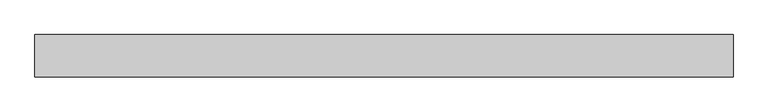
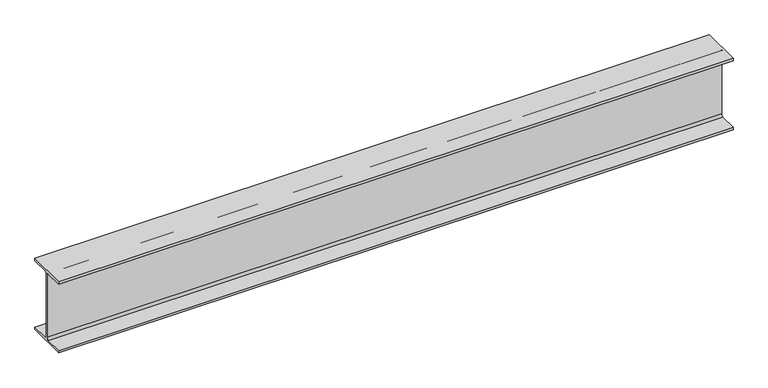
"""IFC4 building model written with IfcOpenShell, lengths in millimetres: beam geometry, Old_Steel Beam_H-KSD3502 : H_SB_ASB_H-194×150x6x9."""

import ifcopenshell
import ifcopenshell.guid

model = None  # the IFC model being written
_history = None  # IfcOwnerHistory: only IFC2X3 demands one
_inside = {}  # id of a spatial element -> (the spatial element, [elements in it])
_under = {}  # id of a project, library or spatial element -> (it, [spatial elements below it])
_declared = {}  # id of a project -> (the project, [libraries it declares])
_typed = {}  # id of a type object -> (the type object, [elements of that type])
_made_of = {}  # id of a material, layer set ... -> (it, [elements and type objects made of it])


def new_model(schema):
    """Start an empty IFC model of exactly this schema.

    Asked for "IFC4X3", IfcOpenShell would pick the latest addendum, in which some entities
    have other attributes; the version numbers below select the first issue.
    IFC2X3 requires an IfcOwnerHistory on every rooted entity: one is made here for all.
    """
    global model, _history
    if schema == "IFC4X3":
        model = ifcopenshell.file(schema_version=(4, 3, 0, 0))
    else:
        model = ifcopenshell.file(schema=schema)
    _inside.clear()
    _under.clear()
    _declared.clear()
    _typed.clear()
    _made_of.clear()
    _history = None
    if model.schema == "IFC2X3":
        org = make("IfcOrganization", Name="unknown")
        user = make(
            "IfcPersonAndOrganization",
            ThePerson=make("IfcPerson", FamilyName="unknown"),
            TheOrganization=org,
        )
        app = make(
            "IfcApplication",
            ApplicationDeveloper=org,
            Version="unknown",
            ApplicationFullName="unknown",
            ApplicationIdentifier="unknown",
        )
        _history = make(
            "IfcOwnerHistory",
            OwningUser=user,
            OwningApplication=app,
            ChangeAction="ADDED",
            CreationDate=0,
        )
    return model


def make(cls, **values):
    """One entity of the class cls with the attributes given. An attribute that is None is left unset."""
    return model.create_entity(
        cls, **{name: value for name, value in values.items() if value is not None}
    )


def rooted(cls, **values):
    """An entity with a GlobalId (a new one), such as an element, a storey or a relation."""
    return make(cls, GlobalId=ifcopenshell.guid.new(), OwnerHistory=_history, **values)


def si_unit(unit_type, name, prefix=None):
    """IfcSIUnit, for example si_unit("LENGTHUNIT", "METRE", prefix="MILLI")."""
    return make("IfcSIUnit", UnitType=unit_type, Prefix=prefix, Name=name)


def assignment(units):
    """IfcUnitAssignment: the units of a project."""
    return None if units is None else make("IfcUnitAssignment", Units=units)


def point(xyz):
    """IfcCartesianPoint."""
    return None if xyz is None else make("IfcCartesianPoint", Coordinates=xyz)


def direction(xyz):
    """IfcDirection."""
    return None if xyz is None else make("IfcDirection", DirectionRatios=xyz)


def frame(location, z_axis=None, x_axis=None):
    """IfcAxis2Placement3D, a coordinate frame: its origin and axes. An axis left out is left unset."""
    return make(
        "IfcAxis2Placement3D",
        Location=point(location),
        Axis=direction(z_axis),
        RefDirection=direction(x_axis),
    )


def frame_2d(location, x_axis=None):
    """IfcAxis2Placement2D, a coordinate frame in the plane: its origin and x axis."""
    return make(
        "IfcAxis2Placement2D", Location=point(location), RefDirection=direction(x_axis)
    )


def origin():
    """The frame at (0, 0, 0) with its axes left unset."""
    return frame((0.0, 0.0, 0.0))


def place(relative_to, where):
    """IfcLocalPlacement: puts the frame where relative to a parent placement (None: the world)."""
    return make(
        "IfcLocalPlacement", PlacementRelTo=relative_to, RelativePlacement=where
    )


def context(
    kind, dimensions, precision=None, world=None, true_north=None, identifier=None
):
    """IfcGeometricRepresentationContext, for example the 3D "Model" context."""
    return make(
        "IfcGeometricRepresentationContext",
        ContextIdentifier=identifier,
        ContextType=kind,
        CoordinateSpaceDimension=dimensions,
        Precision=precision,
        WorldCoordinateSystem=world,
        TrueNorth=true_north,
    )


def project(units=None, contexts=None):
    """IfcProject with its units and contexts."""
    return rooted(
        "IfcProject",
        Name="project",
        RepresentationContexts=contexts,
        UnitsInContext=assignment(units),
    )


def spatial(cls, under=None, at=None, **own):
    """A site, building, storey or space (cls), placed at a placement, below another one or the project."""
    s = rooted(cls, ObjectPlacement=at, **own)
    if under is not None:
        _under.setdefault(under.id(), (under, []))[1].append(s)
    return s


def polyline(points):
    """IfcPolyline through the points."""
    return make("IfcPolyline", Points=[point(p) for p in points])


def circle_curve(where, radius):
    """IfcCircle in the frame where."""
    return make("IfcCircle", Position=where, Radius=radius)


def trimmed(basis, trim1, trim2, sense, master):
    """IfcTrimmedCurve: the piece of a basis curve between two trims."""
    return make(
        "IfcTrimmedCurve",
        BasisCurve=basis,
        Trim1=trim1,
        Trim2=trim2,
        SenseAgreement=sense,
        MasterRepresentation=master,
    )


def segment(curve, same_sense, transition):
    """IfcCompositeCurveSegment."""
    return make(
        "IfcCompositeCurveSegment",
        Transition=transition,
        SameSense=same_sense,
        ParentCurve=curve,
    )


def composite_curve(segments, self_intersect=None):
    """IfcCompositeCurve: segments joined end to end."""
    return make("IfcCompositeCurve", Segments=segments, SelfIntersect=self_intersect)


def outline(outer, holes=None, kind="AREA"):
    """IfcArbitraryClosedProfileDef: a profile drawn as a closed curve; with holes, ...WithVoids."""
    if holes is None:
        return make("IfcArbitraryClosedProfileDef", ProfileType=kind, OuterCurve=outer)
    return make(
        "IfcArbitraryProfileDefWithVoids",
        ProfileType=kind,
        OuterCurve=outer,
        InnerCurves=holes,
    )


def extrude(swept, where, along, depth):
    """IfcExtrudedAreaSolid: the profile swept, set in the frame where, extruded along a direction by depth."""
    return make(
        "IfcExtrudedAreaSolid",
        SweptArea=swept,
        Position=where,
        ExtrudedDirection=direction(along),
        Depth=depth,
    )


def shape(context_of_items, identifier, shape_type, items):
    """IfcShapeRepresentation: the items that make up one representation, for example the "Body"."""
    return make(
        "IfcShapeRepresentation",
        ContextOfItems=context_of_items,
        RepresentationIdentifier=identifier,
        RepresentationType=shape_type,
        Items=items,
    )


def source(mapping_origin, context_of_items, identifier, shape_type, items):
    """IfcRepresentationMap: a shape defined once, which mapped items show again and again."""
    return make(
        "IfcRepresentationMap",
        MappingOrigin=mapping_origin,
        MappedRepresentation=shape(context_of_items, identifier, shape_type, items),
    )


def transform(
    local_origin,
    x_axis=None,
    y_axis=None,
    z_axis=None,
    scale=None,
    scale2=None,
    scale3=None,
    uniform=True,
):
    """IfcCartesianTransformationOperator3D, or its non-uniform kind. x_axis, y_axis, z_axis: its Axis1, 2, 3."""
    if uniform:
        return make(
            "IfcCartesianTransformationOperator3D",
            Axis1=direction(x_axis),
            Axis2=direction(y_axis),
            LocalOrigin=point(local_origin),
            Scale=scale,
            Axis3=direction(z_axis),
        )
    return make(
        "IfcCartesianTransformationOperator3DnonUniform",
        Axis1=direction(x_axis),
        Axis2=direction(y_axis),
        LocalOrigin=point(local_origin),
        Scale=scale,
        Axis3=direction(z_axis),
        Scale2=scale2,
        Scale3=scale3,
    )


def mapped(mapping_source, mapping_target):
    """IfcMappedItem: shows the shape of a source again, moved by a transform."""
    return make(
        "IfcMappedItem", MappingSource=mapping_source, MappingTarget=mapping_target
    )


def made_of(thing, what):
    """Note that an element or type object is made of a material, layer set ...; save() writes the relation."""
    if what is not None:
        _made_of.setdefault(what.id(), (what, []))[1].append(thing)
    return thing


def element(
    cls,
    number,
    at=None,
    inside=None,
    cuts=None,
    type_object=None,
    material=None,
    context=None,
    identifier="Body",
    shape_type=None,
    held_by="IfcProductDefinitionShape",
    body=None,
    shapes=None,
    **own,
):
    """One element of the class cls, such as IfcWall. Its Tag is "e" and its number.

    at: its placement. inside: the storey or other place that contains it. cuts: it is an
    opening in that element (IfcRelVoidsElement). A single representation is given by context,
    identifier, shape_type and body (its items); several are given by shapes. held_by: the class
    of the entity that holds the representations. save() writes the other relations.
    """
    e = rooted(cls, Tag="e%d" % number, ObjectPlacement=at, **own)
    if body is not None:
        shapes = [shape(context, identifier, shape_type, body)]
    if shapes is not None:
        e.Representation = make(held_by, Representations=shapes)
    if inside is not None:
        _inside.setdefault(inside.id(), (inside, []))[1].append(e)
    if cuts is not None:
        rooted(
            "IfcRelVoidsElement", RelatingBuildingElement=cuts, RelatedOpeningElement=e
        )
    if type_object is not None:
        _typed.setdefault(type_object.id(), (type_object, []))[1].append(e)
    return made_of(e, material)


def aggregate(whole, parts):
    """IfcRelAggregates: a whole, such as a stair, and the parts it consists of."""
    return rooted("IfcRelAggregates", RelatingObject=whole, RelatedObjects=parts)


def save(model, path):
    """Write the relations noted so far, then the file.

    IfcRelAggregates (storeys below a building ...), IfcRelContainedInSpatialStructure (elements
    in a storey), IfcRelDefinesByType, IfcRelAssociatesMaterial and IfcRelDeclares: one each for
    every whole, place, type object, material and project.
    """
    for whole, parts in _under.values():
        aggregate(whole, parts)
    for where, things in _inside.values():
        rooted(
            "IfcRelContainedInSpatialStructure",
            RelatedElements=things,
            RelatingStructure=where,
        )
    for kind, things in _typed.values():
        rooted("IfcRelDefinesByType", RelatedObjects=things, RelatingType=kind)
    for what, things in _made_of.values():
        rooted("IfcRelAssociatesMaterial", RelatedObjects=things, RelatingMaterial=what)
    for by, libraries in _declared.values():
        rooted("IfcRelDeclares", RelatingContext=by, RelatedDefinitions=libraries)
    model.write(path)


def beam_e3063bc9(model_context):
    return source(origin(), model_context, "Body", "SweptSolid", [
        extrude(outline(composite_curve([segment(polyline([(-82.5, -141.5), (-11.9, -141.5)]), True, "CONTINUOUS"), segment(trimmed(circle_curve(frame_2d((-11.9, -132.6)), 8.9), [point((-11.9, -141.5))], [point((-3.0, -132.6))], True, "CARTESIAN"), True, "CONTINUOUS"), segment(polyline([(-3.0, -132.6), (-3.0, 132.6)]), True, "CONTINUOUS"), segment(trimmed(circle_curve(frame_2d((-11.9, 132.6)), 8.9), [point((-3.0, 132.6))], [point((-11.9, 141.5))], True, "CARTESIAN"), True, "CONTINUOUS"), segment(polyline([(-11.9, 141.5), (-82.5, 141.5), (-82.5, 151.7), (82.5, 151.7), (82.5, 141.5), (11.9, 141.5)]), True, "CONTINUOUS"), segment(trimmed(circle_curve(frame_2d((11.9, 132.6)), 8.9), [point((11.9, 141.5))], [point((3.0, 132.6))], True, "CARTESIAN"), True, "CONTINUOUS"), segment(polyline([(3.0, 132.6), (3.0, -132.6)]), True, "CONTINUOUS"), segment(trimmed(circle_curve(frame_2d((11.9, -132.6)), 8.9), [point((3.0, -132.6))], [point((11.9, -141.5))], True, "CARTESIAN"), True, "CONTINUOUS"), segment(polyline([(11.9, -141.5), (82.5, -141.5), (82.5, -151.7), (-82.5, -151.7), (-82.5, -141.5)]), True, "CONTINUOUS")], self_intersect=False)), frame((-1579.8617116, 0.0, 0.0), z_axis=(1.0, 0.0, 0.0), x_axis=(0.0, 1.0, 0.0)), (0.0, 0.0, 1.0), 2719.057388),
    ])


if __name__ == "__main__":
    model = new_model("IFC4")
    model_context = context("Model", 3, world=origin())
    ifc_project = project(units=[si_unit("LENGTHUNIT", "METRE", prefix="MILLI")], contexts=[model_context])
    site = spatial("IfcSite", under=ifc_project)
    building = spatial("IfcBuilding", under=site)
    placement = place(None, origin())
    beam_shape = beam_e3063bc9(model_context)
    element("IfcBeam", 1, ObjectType="Old_Steel Beam_H-KSD3502 : H_SB_ASB_H-194×150x6x9", at=placement, inside=building, context=model_context, shape_type="MappedRepresentation", body=[
        mapped(beam_shape, transform((0.0, 0.0, 0.0), x_axis=(1.0, 0.0, 0.0), y_axis=(0.0, 1.0, 0.0), z_axis=(0.0, 0.0, 1.0))),
    ])
    save(model, "model.ifc")

# Revit data of these elements
# Type "Old_Steel Beam_H-KSD3502 : H_SB_ASB_H-194×150x6x9"
#   Width = 15.0 cm
#   Web Thickness = 0.6 cm
#   Web Fillet = 1.3 cm
#   Warping Constant = 43316.0 cm⁶
#   Torsional Moment of Inertia = 8.622 cm⁴
#   Torsional Modulus = 1.0 cm³
#   Section Area = 39.01 cm²
#   Plastic Modulus weak axis = 104.0 cm³
#   Plastic Modulus strong axis = 309.0 cm³
#   Perimeter = 0.95 m²/m
#   Nominal Weight = 30.60 kgf/m
#   Moment of Inertia weak axis = 507.00 cm⁴
#   Moment of Inertia strong axis = 2690.00 cm⁴
#   Height = 19.4 cm
#   Flange Thickness = 0.9 cm
#   Elastic Modulus weak axis = 67.6 cm³
#   Elastic Modulus strong axis = 277.0 cm³
#   Centroid Vertical = 9.7 cm
#   Centroid Horizontal = 7.5 cm
#   Length [instance default] = 1.5240 m
#   Structural Material [instance default] = Steel, 45-345
#   Assembly Code = ""
# Element 1 (IfcBeam, "Old_Steel Beam_H-KSD3502 : H_SB_ASB_H-194×150x6x9")
#   Structural Material = none
# Materials
#   "Steel, 45-345": class "Metal", colour RGB 189 187 185, transparency 0, Description = "Steel 345 MPa", Cost = 0
